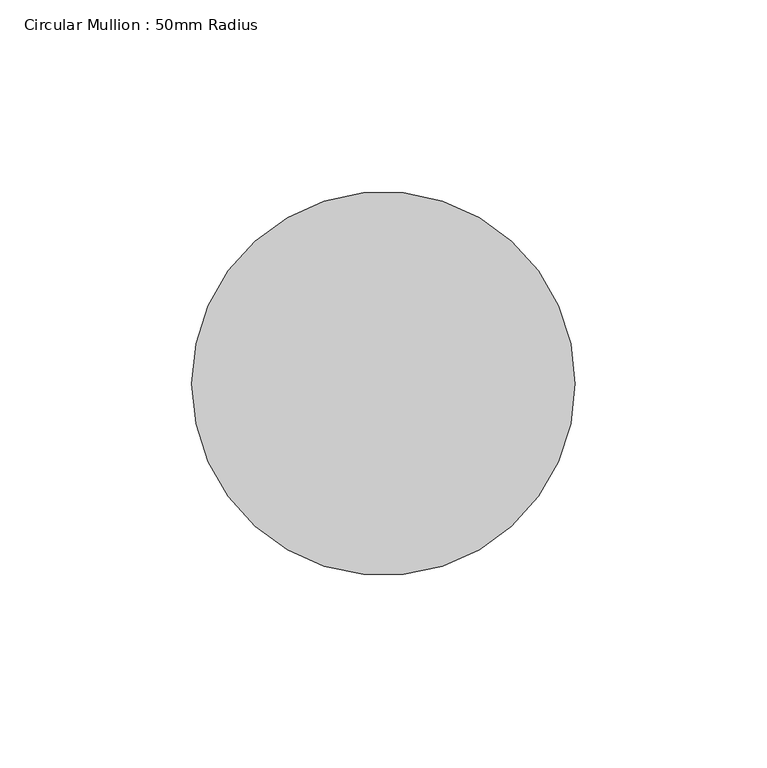
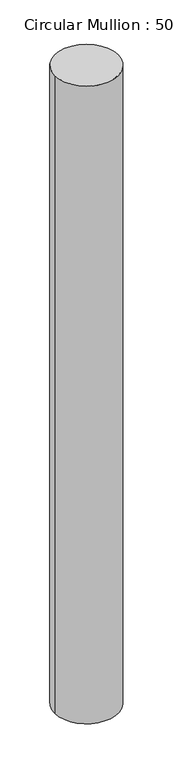
"""IFC4 building model written with IfcOpenShell, lengths in millimetres: member geometry, Circular Mullion : 50mm Radius."""

from ifc_helpers import new_model, si_unit, point, frame, origin, origin_2d, place, context, project, spatial, circle_curve, trimmed, segment, composite_curve, outline, extrude, source, transform, mapped, element, save


def circular_mullion_50mm_radius_5ad49ea9(model_context):
    return source(origin(), model_context, "Body", "SweptSolid", [
        extrude(outline(composite_curve([segment(trimmed(circle_curve(origin_2d(), 50.0), [point((50.0, 0.0))], [point((-50.0, 0.0))], False, "CARTESIAN"), True, "CONTINUOUS"), segment(trimmed(circle_curve(origin_2d(), 50.0), [point((-50.0, 0.0))], [point((50.0, 0.0))], False, "CARTESIAN"), True, "CONTINUOUS")], self_intersect=False)), frame((0.0, 0.0, -1065.3560993), z_axis=(0.0, 0.0, 1.0), x_axis=(1.0, 0.0, 0.0)), (0.0, 0.0, 1.0), 1065.3560993),
    ])


if __name__ == "__main__":
    model = new_model("IFC4")
    model_context = context("Model", 3, world=origin())
    ifc_project = project(units=[si_unit("LENGTHUNIT", "METRE", prefix="MILLI")], contexts=[model_context])
    site = spatial("IfcSite", under=ifc_project)
    building = spatial("IfcBuilding", under=site)
    placement = place(None, origin())
    circular_mullion_50mm_radius_shape = circular_mullion_50mm_radius_5ad49ea9(model_context)
    element("IfcMember", 1, ObjectType="Circular Mullion : 50mm Radius", at=placement, inside=building, context=model_context, shape_type="MappedRepresentation", body=[
        mapped(circular_mullion_50mm_radius_shape, transform((0.0, 0.0, 0.0), x_axis=(1.0, 0.0, 0.0), y_axis=(0.0, 1.0, 0.0), z_axis=(0.0, 0.0, 1.0))),
    ])
    save(model, "model.ifc")

# Revit data of these elements
# Type "Circular Mullion : 50mm Radius"
#   built-in parameter 1007350 = 0.164042 (stored number, unit not read)
# Element 1 (IfcMember, "Circular Mullion : 50mm Radius")
#   Materials on its faces: "Aluminium"
# Materials
#   "Aluminium": class "Metal", colour RGB 247 247 247, transparency 0, Description = "Aluminium 6061", Cost = 0
